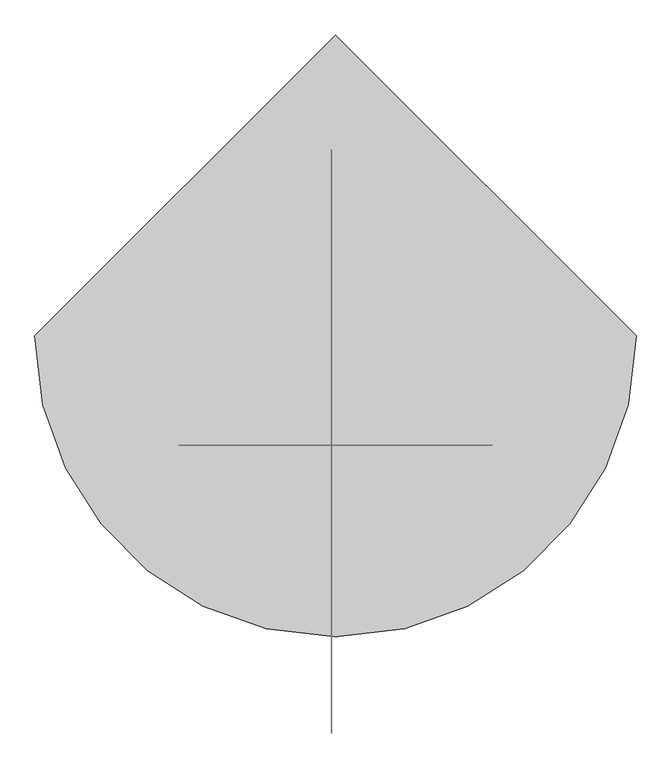
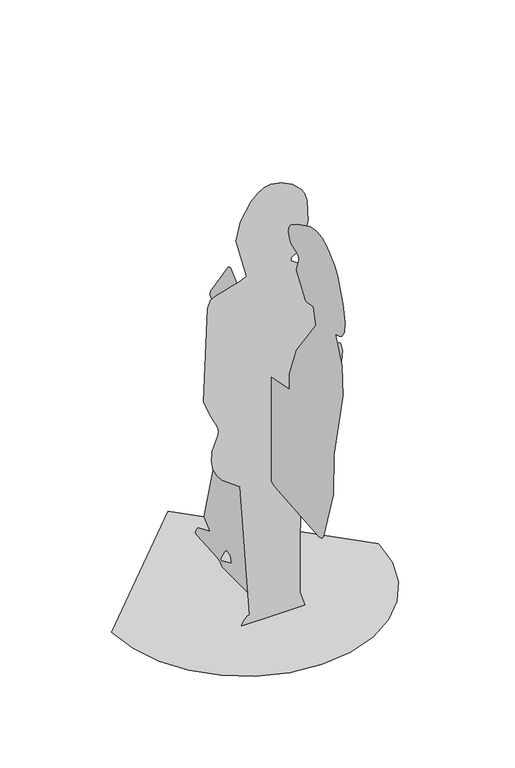
"""IFC4 building model written with IfcOpenShell, lengths in millimetres: proxy geometry, cynthia 25594 : cynthia 25594."""

from ifc_helpers import new_model, si_unit, origin, place, context, project, spatial, triangles, source, transform, mapped, element, save


def entourage_c1b6233a(model_context):
    return source(origin(), model_context, "Body", "Tessellation", [
        triangles([(-437.3057565, 0.0, 2.93e-05), (-425.7448342, -100.2015691, 2.93e-05), (-392.8194094, -192.2206617, 2.93e-05), (-341.1658762, -273.4208834, 2.93e-05), (-273.4209015, -341.1659489, 2.93e-05), (-192.2206254, -392.819373, 2.93e-05), (-100.2015237, -425.7447616, 2.93e-05), (1.91e-05, -437.3057565, 2.93e-05), (100.2015782, -425.7448342, 2.93e-05), (192.220698, -392.8194094, 2.93e-05), (273.4209015, -341.1658762, 2.93e-05), (341.1660215, -273.4209015, 2.93e-05), (392.819373, -192.2206072, 2.93e-05), (425.7447616, -100.2014965, 2.93e-05), (437.3057565, 3.36e-05, 2.93e-05), (-5.73e-05, 437.3057928, 2.93e-05), (-5.5814555, 72.2468665, 69.496344), (-5.5814561, 67.0311374, 46.0256608), (-5.5814578, 124.4039163, 19.9471336), (-5.5814578, 129.6196227, 25.1628196), (-5.5814566, 107.6002182, 62.2269339), (-5.5814561, 95.7175496, 74.7120321), (-5.5814561, -28.6037069, 4.4e-06), (-5.5814549, -39.8908654, 35.5942482), (-5.5814549, -42.4985551, 37.2668205), (-5.5814544, -45.6385706, 39.1827964), (-5.5814544, -48.9915363, 41.1595652), (-5.5814544, -52.2381223, 43.0148345), (-5.5814544, -55.0589122, 44.56573), (-5.5814544, -57.134603, 45.6302408), (-5.5814544, -58.1458059, 46.0256654), (-5.5814555, -58.1458831, 5.3e-06), (-5.5814549, -108.953415, 6.8e-06), (-5.5814538, -116.5758059, 29.8220192), (-5.5814504, -109.3236867, 163.616957), (-5.5814407, -45.4571545, 488.7457126), (-5.5814407, -47.7144295, 510.223653), (-5.5814407, -52.9301177, 512.8314517), (-5.5814402, -176.6935208, 461.1352976), (-5.5814368, -431.0100288, 441.4516153), (-5.5814368, -446.7160832, 445.0272692), (-5.5814362, -456.1585665, 455.8251566), (-5.58143, -511.6809042, 636.0529638), (-5.581426, -514.5202658, 776.2247131), (-5.581418, -566.767113, 1012.4528086), (-5.5814152, -561.4616592, 1112.6378271), (-5.5814129, -522.3438071, 1198.6969637), (-5.5814124, -544.7658397, 1204.5966036), (-5.5814118, -561.2097124, 1214.9815075), (-5.5814112, -573.9143148, 1236.2570984), (-5.5814101, -577.4586843, 1272.8740494), (-5.5814084, -566.4219306, 1329.2823795), (-5.5814067, -535.3830548, 1409.9331253), (-5.5814061, -516.7871696, 1433.7636475), (-5.5814055, -472.5754423, 1474.3203289), (-5.5814055, -445.9831701, 1486.7813416), (-5.5814061, -415.7490054, 1491.187904), (-5.5814067, -381.3846059, 1485.4068615), (-5.5814084, -308.1102267, 1450.1702042), (-5.5814101, -271.6907564, 1426.3735462), (-5.5814101, -259.9822596, 1410.5514015), (-5.5814112, -256.5008769, 1391.3528641), (-5.5814118, -264.1662884, 1368.2074745), (-5.5814118, -270.5525991, 1361.5164585), (-5.5814118, -307.4893707, 1345.9730759), (-5.5814118, -313.689501, 1341.0963387), (-5.5814118, -316.3233155, 1334.3053288), (-5.5814124, -314.5104538, 1321.5896805), (-5.5814141, -303.2841223, 1289.971843), (-5.5814141, -303.9328654, 1281.3184467), (-5.5814146, -344.8551496, 1227.4567635), (-5.5814152, -350.2254976, 1216.9518814), (-5.5814152, -354.0100413, 1213.1371433), (-5.5814152, -360.9104559, 1211.8310457), (-5.5814141, -397.1668548, 1216.9518814), (-5.5814158, -412.8139375, 1162.1869829), (-5.581422, -300.7217424, 1007.464959), (-5.581426, -262.9221964, 903.7018885), (-5.5814271, -261.5584715, 849.2446747), (-5.58143, -151.2454011, 828.1021425), (-5.58143, -131.1657765, 828.3817766), (-5.5814283, -146.9133073, 873.4846922), (-5.5814283, -146.8128955, 875.3230974), (-5.5814283, -136.5283852, 880.5989382), (-5.581426, 66.2908483, 1062.7618017), (-5.581426, 72.9541816, 1068.1172161), (-5.581426, 85.3175848, 1063.7718418), (-5.5814322, 186.9119923, 916.7356859), (-5.5814322, 189.6002729, 904.0094278), (-5.5814339, 74.8547106, 802.3032085), (-5.5814345, 53.5231683, 768.5290346), (-5.5814345, 40.9526102, 757.9697227), (-5.5814345, 7.0502408, 750.1462177), (-5.5814362, -30.739564, 681.3427139), (-5.5814362, -32.0672787, 677.1262562), (-5.5814362, -2.7970168, 673.1418337), (-5.5814379, 74.8547106, 666.6947708), (-5.5814566, 223.5023279, 113.8298525), (-5.5814566, 192.3027424, 86.4272282), (-5.5814566, 189.6002729, 82.5355962), (-5.5814589, 257.4045281, 53.849234), (-5.5814589, 261.0572667, 50.6335418), (-5.5814595, 266.9932052, 41.9573409), (-5.58146, 270.4022813, 33.1798288), (-5.58146, 270.8965462, 29.8373162), (-5.58146, 270.443685, 27.7706614), (-5.58146, 262.21192, 24.6723948), (-5.5814583, 148.3989361, 17.7234776), (-5.5814583, 129.6196227, 12.1235582), (-5.5814583, 119.2279423, 0.0), (-103.2161017, -158.8625234, 3.138314), (-93.5649194, -158.8625234, 19.2429797), (-88.6211895, -158.8625234, 24.4594264), (-82.9717705, -158.8625234, 28.4095146), (-76.7113605, -158.8625234, 30.3784918), (-108.0056077, -158.8625597, 484.1449033), (-166.5178156, -158.8625597, 527.9969141), (-183.6322324, -158.8625597, 549.73316), (-196.1559229, -158.8625597, 575.232294), (-202.0512026, -158.8625597, 604.6165833), (-199.2805142, -158.8625597, 638.0082951), (-180.7337175, -158.8625597, 688.9249546), (-179.5104273, -158.8625597, 700.1737593), (-181.025542, -158.8625597, 711.0281839), (-186.0298695, -158.8625597, 724.8027792), (-192.7431225, -158.8625597, 739.7135696), (-208.5562016, -158.8625597, 771.7148867), (-227.9668628, -158.8625597, 820.5580536), (-215.5926544, -158.8625961, 1139.7188776), (-204.4961842, -158.8625961, 1164.7947453), (-195.70417, -158.8625961, 1170.2243557), (-178.399812, -158.8625961, 1176.5898829), (-156.0960135, -158.8625961, 1183.43634), (-132.3055416, -158.8625961, 1190.3076502), (-110.5412996, -158.8625961, 1196.7492628), (-94.3160908, -158.8625961, 1202.3053917), (-87.1427732, -158.8625961, 1206.520396), (-121.0448735, -158.8625961, 1339.5208534), (-105.9598114, -158.8626324, 1402.4766037), (-72.2006302, -158.8626324, 1459.3927517), (-51.1398881, -158.8626324, 1480.6086079), (-28.7965572, -158.8626324, 1494.3413452), (-6.2993123, -158.8626324, 1498.5999516), (28.3785912, -158.8626324, 1491.3003971), (62.9443683, -158.8626324, 1473.3394295), (92.2084342, -158.8626324, 1445.5309525), (103.2305721, -158.8626324, 1428.187825), (112.1216264, -158.8626324, 1400.9896305), (114.2135136, -158.8625961, 1329.2264236), (96.1614451, -158.8625961, 1258.9090588), (79.8725593, -158.8625961, 1233.5183121), (58.89705, -158.8625961, 1219.5597164), (58.89705, -158.8625961, 1209.1281584), (105.4402574, -158.8625961, 1177.1569994), (186.6818646, -158.8625961, 1146.5396095), (190.9101676, -158.8625961, 1130.2527403), (197.4604945, -158.8625961, 874.5613707), (217.1151996, -158.8625961, 870.6124111), (219.4354431, -158.8625961, 869.5265762), (221.3548754, -158.8625961, 866.986179), (227.9668991, -158.8625597, 839.7665468), (217.9761027, -158.8625597, 726.675412), (216.778683, -158.8625597, 725.5368914), (198.418848, -158.8625597, 721.3532078), (197.1132773, -158.8625597, 721.4595966), (188.2934486, -158.8625597, 736.0849394), (176.2504519, -158.8625597, 750.1460724), (172.5434834, -158.8625597, 744.3783285), (169.4576071, -158.8625597, 737.6237263), (166.7654749, -158.8625597, 730.2866741), (164.2397025, -158.8625597, 722.7717258), (161.6530689, -158.8625597, 715.4834352), (158.7781536, -158.8625597, 708.8262108), (155.3876083, -158.8625597, 703.2046062), (164.5987648, -158.8625597, 582.3864358), (159.7288041, -158.8625597, 557.9936296), (150.1719292, -158.8625597, 536.3020394), (143.452145, -158.8625597, 528.6085773), (105.433708, -158.8625597, 509.5447337), (96.8765541, -158.8625597, 503.2554374), (90.1912608, -158.8625597, 494.5763523), (88.7455914, -158.8625234, 49.4103652), (105.4365966, -158.8625234, 7.4e-05), (-104.3910027, -158.8625234, 7.4e-05)], [[15, 16, 1], [14, 15, 1], [14, 1, 2], [13, 14, 2], [13, 2, 3], [13, 3, 4], [12, 13, 4], [11, 12, 4], [11, 4, 5], [11, 5, 6], [11, 6, 7], [11, 7, 8], [11, 8, 9], [11, 9, 10], [23, 17, 18], [110, 23, 18], [110, 18, 19], [109, 110, 19], [17, 23, 24], [31, 32, 33], [31, 33, 34], [109, 19, 20], [108, 109, 20], [88, 89, 90], [82, 83, 84], [85, 86, 87], [105, 106, 107], [104, 105, 107], [103, 104, 107], [102, 103, 107], [101, 102, 107], [100, 101, 107], [100, 107, 108], [100, 108, 20], [100, 20, 21], [100, 21, 22], [87, 88, 90], [85, 87, 90], [84, 85, 90], [84, 90, 91], [84, 91, 92], [84, 92, 93], [82, 84, 93], [81, 82, 93], [81, 93, 94], [80, 81, 94], [80, 94, 95], [99, 100, 22], [17, 24, 25], [17, 25, 26], [31, 34, 35], [30, 31, 35], [17, 26, 27], [17, 27, 28], [17, 28, 29], [29, 30, 35], [17, 29, 35], [22, 17, 35], [99, 22, 35], [98, 99, 35], [97, 98, 35], [97, 35, 36], [97, 36, 37], [96, 97, 37], [96, 37, 38], [95, 96, 38], [80, 95, 38], [80, 38, 39], [79, 80, 39], [79, 39, 40], [79, 40, 41], [79, 41, 42], [79, 42, 43], [79, 43, 44], [78, 79, 44], [77, 78, 44], [77, 44, 45], [77, 45, 46], [76, 77, 46], [76, 46, 47], [75, 76, 47], [72, 73, 74], [71, 72, 74], [61, 62, 63], [60, 61, 63], [60, 63, 64], [59, 60, 64], [59, 64, 65], [59, 65, 66], [58, 59, 66], [57, 58, 66], [56, 57, 66], [55, 56, 66], [54, 55, 66], [54, 66, 67], [53, 54, 67], [52, 53, 67], [52, 67, 68], [51, 52, 68], [50, 51, 68], [49, 50, 68], [48, 49, 68], [47, 48, 68], [75, 47, 68], [74, 75, 68], [71, 74, 68], [70, 71, 68], [69, 70, 68], [183, 184, 111], [183, 111, 112], [183, 112, 113], [183, 113, 114], [183, 114, 115], [182, 183, 115], [181, 182, 115], [181, 115, 116], [154, 155, 156], [164, 165, 166], [180, 181, 116], [163, 164, 166], [162, 163, 166], [162, 166, 167], [161, 162, 167], [160, 161, 167], [159, 160, 167], [158, 159, 167], [157, 158, 167], [180, 116, 117], [180, 117, 118], [180, 118, 119], [180, 119, 120], [180, 120, 121], [180, 121, 122], [179, 180, 122], [179, 122, 123], [178, 179, 123], [177, 178, 123], [176, 177, 123], [175, 176, 123], [174, 175, 123], [174, 123, 124], [174, 124, 125], [173, 174, 125], [172, 173, 125], [171, 172, 125], [170, 171, 125], [169, 170, 125], [169, 125, 126], [168, 169, 126], [168, 126, 127], [167, 168, 127], [157, 167, 127], [157, 127, 128], [156, 157, 128], [154, 156, 128], [153, 154, 128], [153, 128, 129], [153, 129, 130], [153, 130, 131], [153, 131, 132], [153, 132, 133], [153, 133, 134], [153, 134, 135], [153, 135, 136], [153, 136, 137], [152, 153, 137], [151, 152, 137], [150, 151, 137], [149, 150, 137], [149, 137, 138], [149, 138, 139], [148, 149, 139], [147, 148, 139], [146, 147, 139], [146, 139, 140], [145, 146, 140], [145, 140, 141], [144, 145, 141], [144, 141, 142], [144, 142, 143]], closed=False),
    ])


if __name__ == "__main__":
    model = new_model("IFC4")
    model_context = context("Model", 3, world=origin())
    ifc_project = project(units=[si_unit("LENGTHUNIT", "METRE", prefix="MILLI")], contexts=[model_context])
    site = spatial("IfcSite", under=ifc_project)
    building = spatial("IfcBuilding", under=site)
    placement = place(None, origin())
    entourage_shape = entourage_c1b6233a(model_context)
    element("IfcBuildingElementProxy", 1, Name="cynthia 25594 : cynthia 25594", ObjectType="cynthia 25594 : cynthia 25594", at=placement, inside=building, context=model_context, shape_type="MappedRepresentation", body=[
        mapped(entourage_shape, transform((0.0, 0.0, 0.0), x_axis=(1.0, 0.0, 0.0), y_axis=(0.0, 1.0, 0.0), z_axis=(0.0, 0.0, 1.0))),
    ])
    save(model, "model.ifc")

# Revit data of these elements
# Type "cynthia 25594 : cynthia 25594"
#   built-in parameter 1005195 = "RPC-8-FXA2-QQQ0-UGV2-6"
#   Height = 0
